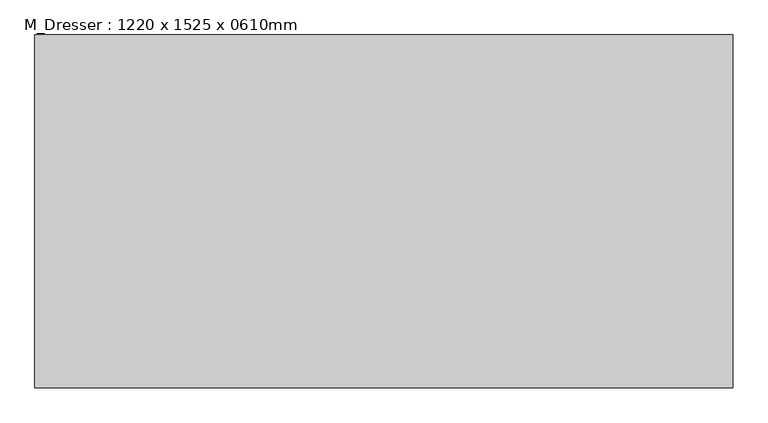
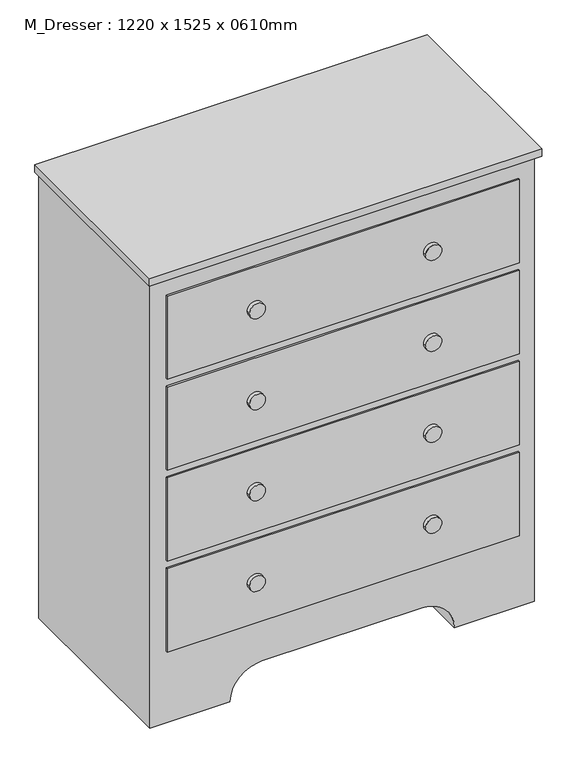
"""IFC4 building model written with IfcOpenShell, lengths in millimetres: furniture geometry, M_Dresser : 1220 x 1525 x 0610mm."""

from ifc_helpers import new_model, si_unit, point, frame, frame_2d, origin, place, context, project, spatial, polyline, circle_curve, trimmed, segment, composite_curve, outline, extrude, source, transform, mapped, element, save


def m_dresser_1220_x_1525_x_0610mm_18e1f140(model_context):
    return source(origin(), model_context, "Body", "SweptSolid", [
        extrude(outline(polyline([(353.5067402, -58.1629541), (353.5067402, -687.2129541), (-891.8932598, -687.2129541), (-891.8932598, -58.1629541), (353.5067402, -58.1629541)])), frame((0.0, 0.0, 1499.6), z_axis=(0.0, 0.0, 1.0), x_axis=(1.0, 0.0, 0.0)), (0.0, 0.0, 1.0), 25.4),
        extrude(outline(composite_curve([segment(polyline([(0.0, 340.8067402), (1499.6, 340.8067402), (1499.6, -879.1932598), (0.0, -879.1932598), (0.0, -625.1932598)]), True, "CONTINUOUS"), segment(trimmed(circle_curve(frame_2d((0.0, -523.5932598)), 101.6), [point((0.0, -625.1932598))], [point((101.6, -523.5932598))], True, "CARTESIAN"), True, "CONTINUOUS"), segment(polyline([(101.6, -523.5932598), (101.6, -14.7932598)]), True, "CONTINUOUS"), segment(trimmed(circle_curve(frame_2d((0.0, -14.7932598)), 101.6), [point((101.6, -14.7932598))], [point((0.0, 86.8067402))], True, "CARTESIAN"), True, "CONTINUOUS"), segment(polyline([(0.0, 86.8067402), (0.0, 340.8067402)]), True, "CONTINUOUS")], self_intersect=False)), frame((0.0, -668.1629541, 0.0), z_axis=(0.0, 1.0, 0.0), x_axis=(0.0, 0.0, 1.0)), (0.0, 0.0, 1.0), 610.0),
        extrude(outline(composite_curve([segment(trimmed(circle_curve(frame_2d((1296.275, 10.4067402)), 25.4), [point((1296.275, -14.9932598))], [point((1296.275, 35.8067402))], False, "CARTESIAN"), True, "CONTINUOUS"), segment(trimmed(circle_curve(frame_2d((1296.275, 10.4067402)), 25.4), [point((1296.275, 35.8067402))], [point((1296.275, -14.9932598))], False, "CARTESIAN"), True, "CONTINUOUS")], self_intersect=False)), frame((0.0, -687.2129541, 0.0), z_axis=(0.0, 1.0, 0.0), x_axis=(0.0, 0.0, 1.0)), (0.0, 0.0, 1.0), 12.7),
        extrude(outline(composite_curve([segment(trimmed(circle_curve(frame_2d((991.225, 10.4067402)), 25.4), [point((991.225, -14.9932598))], [point((991.225, 35.8067402))], False, "CARTESIAN"), True, "CONTINUOUS"), segment(trimmed(circle_curve(frame_2d((991.225, 10.4067402)), 25.4), [point((991.225, 35.8067402))], [point((991.225, -14.9932598))], False, "CARTESIAN"), True, "CONTINUOUS")], self_intersect=False)), frame((0.0, -687.2129541, 0.0), z_axis=(0.0, 1.0, 0.0), x_axis=(0.0, 0.0, 1.0)), (0.0, 0.0, 1.0), 12.7),
        extrude(outline(composite_curve([segment(trimmed(circle_curve(frame_2d((686.175, 10.4067402)), 25.4), [point((686.175, -14.9932598))], [point((686.175, 35.8067402))], False, "CARTESIAN"), True, "CONTINUOUS"), segment(trimmed(circle_curve(frame_2d((686.175, 10.4067402)), 25.4), [point((686.175, 35.8067402))], [point((686.175, -14.9932598))], False, "CARTESIAN"), True, "CONTINUOUS")], self_intersect=False)), frame((0.0, -687.2129541, 0.0), z_axis=(0.0, 1.0, 0.0), x_axis=(0.0, 0.0, 1.0)), (0.0, 0.0, 1.0), 12.7),
        extrude(outline(composite_curve([segment(trimmed(circle_curve(frame_2d((381.125, 10.4067402)), 25.4), [point((381.125, -14.9932598))], [point((381.125, 35.8067402))], False, "CARTESIAN"), True, "CONTINUOUS"), segment(trimmed(circle_curve(frame_2d((381.125, 10.4067402)), 25.4), [point((381.125, 35.8067402))], [point((381.125, -14.9932598))], False, "CARTESIAN"), True, "CONTINUOUS")], self_intersect=False)), frame((0.0, -687.2129541, 0.0), z_axis=(0.0, 1.0, 0.0), x_axis=(0.0, 0.0, 1.0)), (0.0, 0.0, 1.0), 12.7),
        extrude(outline(composite_curve([segment(trimmed(circle_curve(frame_2d((381.125, -548.7932598)), 25.4), [point((381.125, -574.1932598))], [point((381.125, -523.3932598))], False, "CARTESIAN"), True, "CONTINUOUS"), segment(trimmed(circle_curve(frame_2d((381.125, -548.7932598)), 25.4), [point((381.125, -523.3932598))], [point((381.125, -574.1932598))], False, "CARTESIAN"), True, "CONTINUOUS")], self_intersect=False)), frame((0.0, -687.2129541, 0.0), z_axis=(0.0, 1.0, 0.0), x_axis=(0.0, 0.0, 1.0)), (0.0, 0.0, 1.0), 12.7),
        extrude(outline(composite_curve([segment(trimmed(circle_curve(frame_2d((686.175, -548.7932598)), 25.4), [point((686.175, -574.1932598))], [point((686.175, -523.3932598))], False, "CARTESIAN"), True, "CONTINUOUS"), segment(trimmed(circle_curve(frame_2d((686.175, -548.7932598)), 25.4), [point((686.175, -523.3932598))], [point((686.175, -574.1932598))], False, "CARTESIAN"), True, "CONTINUOUS")], self_intersect=False)), frame((0.0, -687.2129541, 0.0), z_axis=(0.0, 1.0, 0.0), x_axis=(0.0, 0.0, 1.0)), (0.0, 0.0, 1.0), 12.7),
        extrude(outline(composite_curve([segment(trimmed(circle_curve(frame_2d((991.225, -548.7932598)), 25.4), [point((991.225, -574.1932598))], [point((991.225, -523.3932598))], False, "CARTESIAN"), True, "CONTINUOUS"), segment(trimmed(circle_curve(frame_2d((991.225, -548.7932598)), 25.4), [point((991.225, -523.3932598))], [point((991.225, -574.1932598))], False, "CARTESIAN"), True, "CONTINUOUS")], self_intersect=False)), frame((0.0, -687.2129541, 0.0), z_axis=(0.0, 1.0, 0.0), x_axis=(0.0, 0.0, 1.0)), (0.0, 0.0, 1.0), 12.7),
        extrude(outline(composite_curve([segment(trimmed(circle_curve(frame_2d((1296.275, -548.7932598)), 25.4), [point((1296.275, -574.1932598))], [point((1296.275, -523.3932598))], False, "CARTESIAN"), True, "CONTINUOUS"), segment(trimmed(circle_curve(frame_2d((1296.275, -548.7932598)), 25.4), [point((1296.275, -523.3932598))], [point((1296.275, -574.1932598))], False, "CARTESIAN"), True, "CONTINUOUS")], self_intersect=False)), frame((0.0, -687.2129541, 0.0), z_axis=(0.0, 1.0, 0.0), x_axis=(0.0, 0.0, 1.0)), (0.0, 0.0, 1.0), 12.7),
        extrude(outline(polyline([(290.0067402, -674.5129541), (-828.3932598, -674.5129541), (-828.3932598, -668.1629541), (290.0067402, -668.1629541), (290.0067402, -674.5129541)])), frame((0.0, 0.0, 1156.45), z_axis=(0.0, 0.0, 1.0), x_axis=(1.0, 0.0, 0.0)), (0.0, 0.0, 1.0), 279.65),
        extrude(outline(polyline([(290.0067402, -674.5129541), (-828.3932598, -674.5129541), (-828.3932598, -668.1629541), (290.0067402, -668.1629541), (290.0067402, -674.5129541)])), frame((0.0, 0.0, 851.4), z_axis=(0.0, 0.0, 1.0), x_axis=(1.0, 0.0, 0.0)), (0.0, 0.0, 1.0), 279.65),
        extrude(outline(polyline([(290.0067402, -674.5129541), (-828.3932598, -674.5129541), (-828.3932598, -668.1629541), (290.0067402, -668.1629541), (290.0067402, -674.5129541)])), frame((0.0, 0.0, 546.35), z_axis=(0.0, 0.0, 1.0), x_axis=(1.0, 0.0, 0.0)), (0.0, 0.0, 1.0), 279.65),
        extrude(outline(polyline([(290.0067402, -674.5129541), (-828.3932598, -674.5129541), (-828.3932598, -668.1629541), (290.0067402, -668.1629541), (290.0067402, -674.5129541)])), frame((0.0, 0.0, 241.3), z_axis=(0.0, 0.0, 1.0), x_axis=(1.0, 0.0, 0.0)), (0.0, 0.0, 1.0), 279.65),
    ])


if __name__ == "__main__":
    model = new_model("IFC4")
    model_context = context("Model", 3, world=origin())
    ifc_project = project(units=[si_unit("LENGTHUNIT", "METRE", prefix="MILLI")], contexts=[model_context])
    site = spatial("IfcSite", under=ifc_project)
    building = spatial("IfcBuilding", under=site)
    placement = place(None, origin())
    m_dresser_1220_x_1525_x_0610mm_shape = m_dresser_1220_x_1525_x_0610mm_18e1f140(model_context)
    element("IfcFurniture", 1, ObjectType="M_Dresser : 1220 x 1525 x 0610mm", at=placement, inside=building, context=model_context, shape_type="MappedRepresentation", body=[
        mapped(m_dresser_1220_x_1525_x_0610mm_shape, transform((0.0, 0.0, 0.0), x_axis=(1.0, 0.0, 0.0), y_axis=(0.0, 1.0, 0.0), z_axis=(0.0, 0.0, 1.0))),
    ])
    save(model, "model.ifc")

# Revit data of these elements
# Type "M_Dresser : 1220 x 1525 x 0610mm"
#   Depth = 0.61 m
#   Height = 1.525 m
#   Width = 1.22 m
#   Dresser Material = Laminate - Ivory, Glossy
#   Drawer Material = Laminate, Ivory, Matte
#   Knob Material = Cherry
#   Default Elevation = 0
# Element 1 (IfcFurniture, "M_Dresser : 1220 x 1525 x 0610mm")
#   Materials on its faces: "Laminate, Ivory, Matte", "Cherry", "Laminate - Ivory, Glossy"
# Materials
#   "Laminate - Ivory, Glossy": class "Miscellaneous", colour RGB 247 247 239, transparency 0
#   "Laminate, Ivory, Matte": class "Plastic", colour RGB 247 247 229, transparency 0, Description = "Plastic Laminate - Ivory, Matte", Cost = 0
#   "Cherry": class "Wood", colour RGB 157 77 38, transparency 0, Description = "Prunus Serotina", Cost = 0
